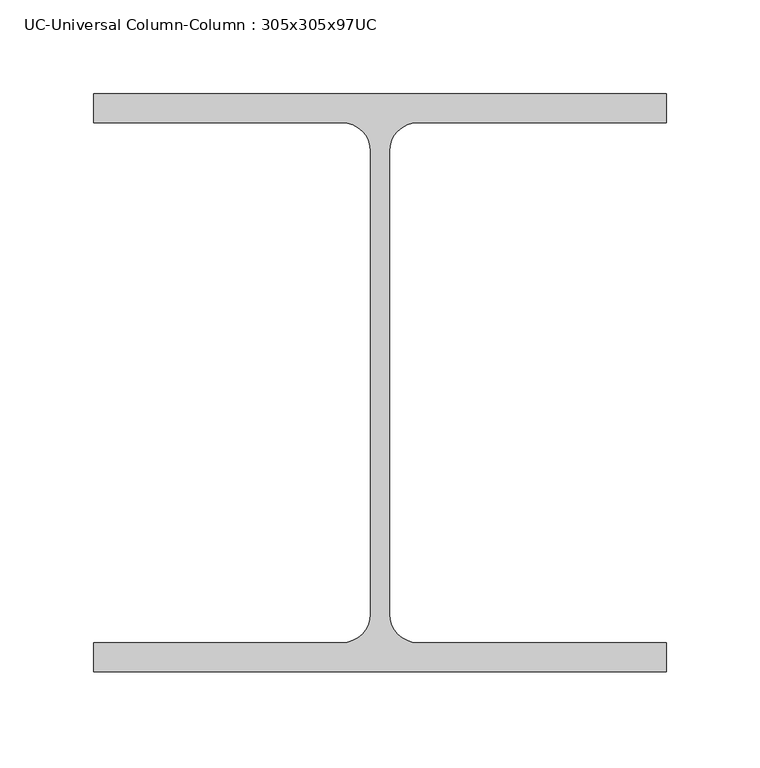
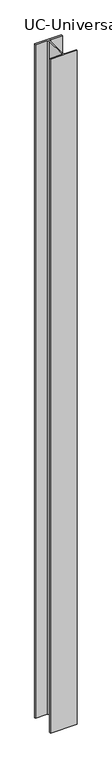
"""IFC4 building model written with IfcOpenShell, lengths in millimetres: column geometry, UC-Universal Column-Column : 305x305x97UC."""

from ifc_helpers import new_model, si_unit, point, frame, frame_2d, origin, place, context, project, spatial, polyline, circle_curve, trimmed, segment, composite_curve, outline, extrude, source, transform, mapped, element, save


def uc_universal_column_column_305x305x97uc_43a052ce(model_context):
    return source(origin(), model_context, "Body", "SweptSolid", [
        extrude(outline(composite_curve([segment(polyline([(152.65, 153.95), (152.65, 138.55), (20.15, 138.55)]), True, "CONTINUOUS"), segment(trimmed(circle_curve(frame_2d((20.15, 123.35)), 15.2), [point((20.15, 138.55))], [point((4.95, 123.35))], True, "CARTESIAN"), True, "CONTINUOUS"), segment(polyline([(4.95, 123.35), (4.95, -123.35)]), True, "CONTINUOUS"), segment(trimmed(circle_curve(frame_2d((20.15, -123.35)), 15.2), [point((4.95, -123.35))], [point((20.15, -138.55))], True, "CARTESIAN"), True, "CONTINUOUS"), segment(polyline([(20.15, -138.55), (152.65, -138.55), (152.65, -153.95), (-152.65, -153.95), (-152.65, -138.55), (-20.15, -138.55)]), True, "CONTINUOUS"), segment(trimmed(circle_curve(frame_2d((-20.15, -123.35)), 15.2), [point((-20.15, -138.55))], [point((-4.95, -123.35))], True, "CARTESIAN"), True, "CONTINUOUS"), segment(polyline([(-4.95, -123.35), (-4.95, 123.35)]), True, "CONTINUOUS"), segment(trimmed(circle_curve(frame_2d((-20.15, 123.35)), 15.2), [point((-4.95, 123.35))], [point((-20.15, 138.55))], True, "CARTESIAN"), True, "CONTINUOUS"), segment(polyline([(-20.15, 138.55), (-152.65, 138.55), (-152.65, 153.95), (152.65, 153.95)]), True, "CONTINUOUS")], self_intersect=False)), frame((0.0, 0.0, -1500.0), z_axis=(0.0, 0.0, 1.0), x_axis=(1.0, 0.0, 0.0)), (0.0, 0.0, 1.0), 8100.0),
    ])


if __name__ == "__main__":
    model = new_model("IFC4")
    model_context = context("Model", 3, world=origin())
    ifc_project = project(units=[si_unit("LENGTHUNIT", "METRE", prefix="MILLI")], contexts=[model_context])
    site = spatial("IfcSite", under=ifc_project)
    building = spatial("IfcBuilding", under=site)
    placement = place(None, origin())
    uc_universal_column_column_305x305x97uc_shape = uc_universal_column_column_305x305x97uc_43a052ce(model_context)
    element("IfcColumn", 1, ObjectType="UC-Universal Column-Column : 305x305x97UC", at=placement, inside=building, context=model_context, shape_type="MappedRepresentation", body=[
        mapped(uc_universal_column_column_305x305x97uc_shape, transform((0.0, 0.0, 0.0), x_axis=(1.0, 0.0, 0.0), y_axis=(0.0, 1.0, 0.0), z_axis=(0.0, 0.0, 1.0))),
    ])
    save(model, "model.ifc")

# Revit data of these elements
# Type "UC-Universal Column-Column : 305x305x97UC"
#   Keynote = "G10"
#   Nominal h = ""
#   W = 0
#   Ix = 0
#   M = 96.9
#   Zx = 0
#   b = 305.3 mm
#   h = 307.9 mm
#   r = 15.2 mm
#   s = 9.9 mm
#   t = 15.4 mm
#   A = 123 m²
#   Structural Material [instance default] = Steel, 45-345
#   Assembly Code = ""
# Element 1 (IfcColumn, "UC-Universal Column-Column : 305x305x97UC")
#   Materials on its faces: "Steel, 45-345"
# Materials
#   "Steel, 45-345": class "Metal", colour RGB 247 247 247, transparency 0, Description = "Steel 345 MPa", Cost = 0
